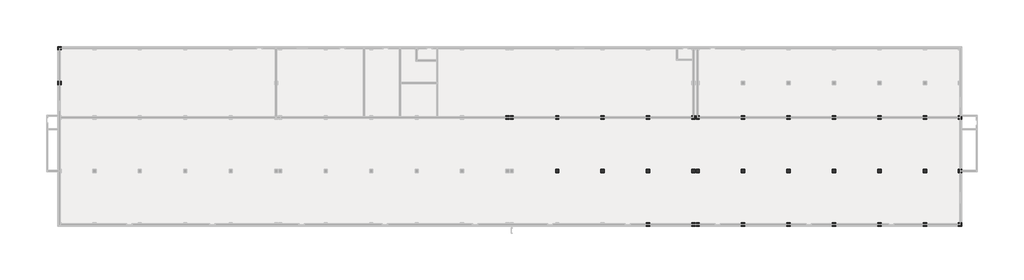
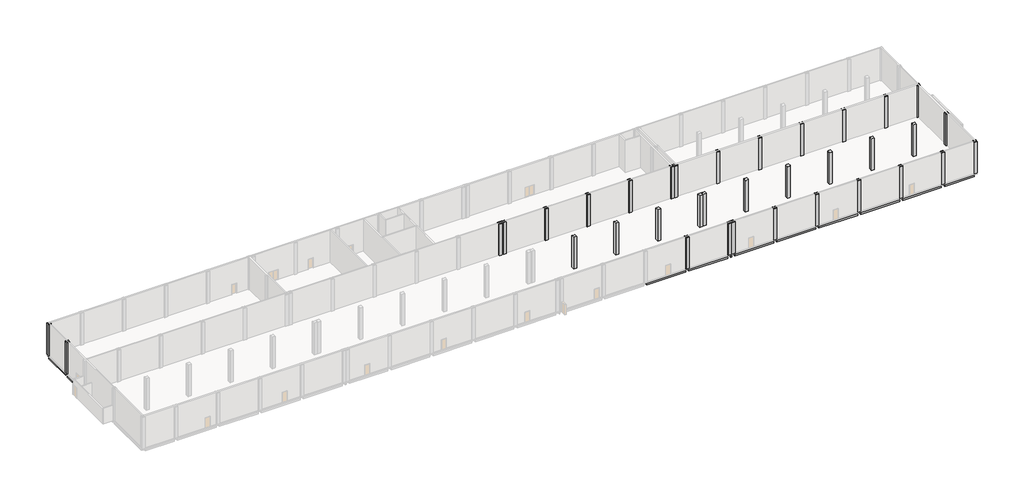
# One storey, part 3 of 4: 35 columns, 13 beams.
"""IFC4 building model written with IfcOpenShell, lengths in millimetres."""

from ifc_helpers import new_model, si_unit, frame, origin, place, context, project, spatial, polyline, outline, extrude, faceted_brep, element, save

model = new_model("IFC4")

# Units and contexts
model_context = context("Model", 3, world=origin())
ifc_project = project(units=[si_unit("LENGTHUNIT", "METRE", prefix="MILLI")], contexts=[model_context])

# Site, building, storey
site = spatial("IfcSite", under=ifc_project)
building = spatial("IfcBuilding", under=site)
storey = spatial("IfcBuildingStorey", under=building, Name="01_T.O.F", Elevation=299.9618634)

# Beams
placement = place(None, origin())
element("IfcBeam", 1, ObjectType="RC Beam_Rectangular : H_SB_AR_S16_TG_B400xH600", at=placement, inside=storey, context=model_context, shape_type="SweptSolid", body=[
    extrude(outline(polyline([(157955.0, -6300.4791411), (158305.0, -6300.4791411), (158305.0, -15350.4791411), (157955.0, -15350.4791411), (157955.0, -6300.4791411)])), frame((0.0, 0.0, -300.0381366), z_axis=(0.0, 0.0, 1.0), x_axis=(1.0, 0.0, 0.0)), (0.0, 0.0, 1.0), 450.0),
])
element("IfcBeam", 2, ObjectType="RC Beam_Rectangular : H_SB_AR_S16_TG_B400xH600", at=placement, inside=storey, context=model_context, shape_type="SweptSolid", body=[
    extrude(outline(polyline([(157955.0, -15950.4791411), (158305.0, -15950.4791411), (158305.0, -25000.4791411), (157955.0, -25000.4791411), (157955.0, -15950.4791411)])), frame((0.0, 0.0, -300.0381366), z_axis=(0.0, 0.0, 1.0), x_axis=(1.0, 0.0, 0.0)), (0.0, 0.0, 1.0), 450.0),
])
element("IfcBeam", 3, ObjectType="RC Beam_Rectangular : H_SB_AR_S16_TG_B400xH600", at=placement, inside=storey, context=model_context, shape_type="SweptSolid", body=[
    extrude(outline(polyline([(-4195.0, 549.5208589), (-4545.0, 549.5208589), (-4545.0, 6199.5208589), (-4195.0, 6199.5208589), (-4195.0, 549.5208589)])), frame((0.0, 0.0, -300.0381366), z_axis=(0.0, 0.0, 1.0), x_axis=(1.0, 0.0, 0.0)), (0.0, 0.0, 1.0), 450.0),
])
element("IfcBeam", 4, ObjectType="RC Beam_Rectangular : H_SB_AR_S16_TG_B400xH600", at=placement, inside=storey, context=model_context, shape_type="SweptSolid", body=[
    extrude(outline(polyline([(-4545.0, -50.4791411), (-4195.0, -50.4791411), (-4195.0, -5700.4791411), (-4545.0, -5700.4791411), (-4545.0, -50.4791411)])), frame((0.0, 0.0, -300.0381366), z_axis=(0.0, 0.0, 1.0), x_axis=(1.0, 0.0, 0.0)), (0.0, 0.0, 1.0), 450.0),
])
element("IfcBeam", 5, ObjectType="RC Beam_Rectangular : H_SB_AR_S16_TG_B400xH600", at=placement, inside=storey, context=model_context, shape_type="SweptSolid", body=[
    extrude(outline(polyline([(93930.0, -25475.4791411), (93930.0, -25125.4791411), (101530.0, -25125.4791411), (101530.0, -25475.4791411), (93930.0, -25475.4791411)])), frame((0.0, 0.0, -300.0381366), z_axis=(0.0, 0.0, 1.0), x_axis=(1.0, 0.0, 0.0)), (0.0, 0.0, 1.0), 450.0),
])
element("IfcBeam", 6, ObjectType="RC Beam_Rectangular : H_SB_AR_S16_TG_B400xH600", at=placement, inside=storey, context=model_context, shape_type="SweptSolid", body=[
    extrude(outline(polyline([(102130.0, -25475.4791411), (102130.0, -25125.4791411), (109730.0, -25125.4791411), (109730.0, -25475.4791411), (102130.0, -25475.4791411)])), frame((0.0, 0.0, -300.0381366), z_axis=(0.0, 0.0, 1.0), x_axis=(1.0, 0.0, 0.0)), (0.0, 0.0, 1.0), 450.0),
])
element("IfcBeam", 7, ObjectType="RC Beam_Rectangular : H_SB_AR_S16_TG_B400xH600", at=placement, inside=storey, context=model_context, shape_type="SweptSolid", body=[
    extrude(outline(polyline([(110330.0, -25475.4791411), (110330.0, -25125.4791411), (110480.0, -25125.4791411), (110480.0, -25475.4791411), (110330.0, -25475.4791411)])), frame((0.0, 0.0, -300.0381366), z_axis=(0.0, 0.0, 1.0), x_axis=(1.0, 0.0, 0.0)), (0.0, 0.0, 1.0), 450.0),
])
element("IfcBeam", 8, ObjectType="RC Beam_Rectangular : H_SB_AR_S16_TG_B400xH600", at=placement, inside=storey, context=model_context, shape_type="SweptSolid", body=[
    extrude(outline(polyline([(111080.0, -25475.4791411), (111080.0, -25125.4791411), (118680.0, -25125.4791411), (118680.0, -25475.4791411), (111080.0, -25475.4791411)])), frame((0.0, 0.0, -300.0381366), z_axis=(0.0, 0.0, 1.0), x_axis=(1.0, 0.0, 0.0)), (0.0, 0.0, 1.0), 450.0),
])
element("IfcBeam", 9, ObjectType="RC Beam_Rectangular : H_SB_AR_S16_TG_B400xH600", at=placement, inside=storey, context=model_context, shape_type="SweptSolid", body=[
    extrude(outline(polyline([(119280.0, -25475.4791411), (119280.0, -25125.4791411), (126880.0, -25125.4791411), (126880.0, -25475.4791411), (119280.0, -25475.4791411)])), frame((0.0, 0.0, -300.0381366), z_axis=(0.0, 0.0, 1.0), x_axis=(1.0, 0.0, 0.0)), (0.0, 0.0, 1.0), 450.0),
])
element("IfcBeam", 10, ObjectType="RC Beam_Rectangular : H_SB_AR_S16_TG_B400xH600", at=placement, inside=storey, context=model_context, shape_type="SweptSolid", body=[
    extrude(outline(polyline([(127480.0, -25475.4791411), (127480.0, -25125.4791411), (135080.0, -25125.4791411), (135080.0, -25475.4791411), (127480.0, -25475.4791411)])), frame((0.0, 0.0, -300.0381366), z_axis=(0.0, 0.0, 1.0), x_axis=(1.0, 0.0, 0.0)), (0.0, 0.0, 1.0), 450.0),
])
element("IfcBeam", 11, ObjectType="RC Beam_Rectangular : H_SB_AR_S16_TG_B400xH600", at=placement, inside=storey, context=model_context, shape_type="SweptSolid", body=[
    extrude(outline(polyline([(135680.0, -25475.4791411), (135680.0, -25125.4791411), (143280.0, -25125.4791411), (143280.0, -25475.4791411), (135680.0, -25475.4791411)])), frame((0.0, 0.0, -300.0381366), z_axis=(0.0, 0.0, 1.0), x_axis=(1.0, 0.0, 0.0)), (0.0, 0.0, 1.0), 450.0),
])
element("IfcBeam", 12, ObjectType="RC Beam_Rectangular : H_SB_AR_S16_TG_B400xH600", at=placement, inside=storey, context=model_context, shape_type="SweptSolid", body=[
    extrude(outline(polyline([(143880.0, -25475.4791411), (143880.0, -25125.4791411), (151480.0, -25125.4791411), (151480.0, -25475.4791411), (143880.0, -25475.4791411)])), frame((0.0, 0.0, -300.0381366), z_axis=(0.0, 0.0, 1.0), x_axis=(1.0, 0.0, 0.0)), (0.0, 0.0, 1.0), 450.0),
])
element("IfcBeam", 13, ObjectType="RC Beam_Rectangular : H_SB_AR_S16_TG_B400xH600", at=placement, inside=storey, context=model_context, shape_type="SweptSolid", body=[
    extrude(outline(polyline([(152080.0, -25475.4791411), (152080.0, -25125.4791411), (157830.0, -25125.4791411), (157830.0, -25475.4791411), (152080.0, -25475.4791411)])), frame((0.0, 0.0, -300.0381366), z_axis=(0.0, 0.0, 1.0), x_axis=(1.0, 0.0, 0.0)), (0.0, 0.0, 1.0), 450.0),
])

# Columns
element("IfcColumn", 14, ObjectType="RC_Column_Rectangular : H_SC_AR_S15_W600xL600", at=placement, inside=storey, context=model_context, shape_type="Brep", body=[
    faceted_brep([(-4070.0, 549.5208589, 299.9618634), (-4070.0, -50.4791411, 299.9618634), (-4670.0, -50.4791411, 299.9618634), (-4670.0, 549.5208589, 299.9618634), (-4070.0, 549.5208589, 6848.9618634), (-4070.0, 399.5208589, 6848.9618634), (-4070.0, 99.5208589, 6848.9618634), (-4070.0, -50.4791411, 6848.9618634), (-4220.0, -50.4791411, 6848.9618634), (-4520.0, -50.4791411, 6848.9618634), (-4670.0, -50.4791411, 6848.9618634), (-4670.0, 549.5208589, 6848.9618634), (-4520.0, 549.5208589, 6848.9618634), (-4220.0, 549.5208589, 6848.9618634)], [[[0, 1, 2, 3]], [[1, 0, 4, 5, 6, 7]], [[2, 1, 7, 8, 9, 10]], [[3, 2, 10, 11]], [[0, 3, 11, 12, 13, 4]], [[7, 6, 5, 4, 13, 12, 11, 10, 9, 8]]]),
])
element("IfcColumn", 15, ObjectType="RC_Column_Rectangular : H_SC_AR_S15_W600xL600", at=placement, inside=storey, context=model_context, shape_type="Brep", body=[
    faceted_brep([(-4070.0, 6799.5208589, 299.9618634), (-4070.0, 6199.5208589, 299.9618634), (-4670.0, 6199.5208589, 299.9618634), (-4670.0, 6799.5208589, 299.9618634), (-4070.0, 6799.5208589, 6848.9618634), (-4070.0, 6649.5208589, 6848.9618634), (-4070.0, 6349.5208589, 6848.9618634), (-4070.0, 6199.5208589, 6848.9618634), (-4220.0, 6199.5208589, 6848.9618634), (-4520.0, 6199.5208589, 6848.9618634), (-4670.0, 6199.5208589, 6848.9618634), (-4670.0, 6799.5208589, 6848.9618634)], [[[0, 1, 2, 3]], [[1, 0, 4, 5, 6, 7]], [[2, 1, 7, 8, 9, 10]], [[3, 2, 10, 11]], [[0, 3, 11, 4]], [[7, 6, 5, 4, 11, 10, 9, 8]]]),
])
element("IfcColumn", 16, ObjectType="RC_Column_Rectangular : H_SC_AR_S15_W600xL600", at=placement, inside=storey, context=model_context, shape_type="Brep", body=[
    faceted_brep([(76780.0, -5700.4791411, 299.9618634), (76780.0, -6300.4791411, 299.9618634), (76180.0, -6300.4791411, 299.9618634), (76180.0, -5700.4791411, 299.9618634), (76780.0, -5700.4791411, 6848.9618634), (76780.0, -5850.4791411, 6848.9618634), (76780.0, -6150.4791411, 6848.9618634), (76780.0, -6300.4791411, 6848.9618634), (76630.0, -6300.4791411, 6848.9618634), (76330.0, -6300.4791411, 6848.9618634), (76180.0, -6300.4791411, 6848.9618634), (76180.0, -6150.4791411, 6848.9618634), (76180.0, -5850.4791411, 6848.9618634), (76180.0, -5700.4791411, 6848.9618634), (76330.0, -5700.4791411, 6848.9618634), (76630.0, -5700.4791411, 6848.9618634)], [[[0, 1, 2, 3]], [[1, 0, 4, 5, 6, 7]], [[2, 1, 7, 8, 9, 10]], [[3, 2, 10, 11, 12, 13]], [[0, 3, 13, 14, 15, 4]], [[7, 6, 5, 4, 15, 14, 13, 12, 11, 10, 9, 8]]]),
])
element("IfcColumn", 17, ObjectType="RC_Column_Rectangular : H_SC_AR_S15_W600xL600", at=placement, inside=storey, context=model_context, shape_type="Brep", body=[
    faceted_brep([(77530.0, -5700.4791411, 299.9618634), (77530.0, -6300.4791411, 299.9618634), (76930.0, -6300.4791411, 299.9618634), (76930.0, -5700.4791411, 299.9618634), (77530.0, -5700.4791411, 6848.9618634), (77530.0, -5850.4791411, 6848.9618634), (77530.0, -6150.4791411, 6848.9618634), (77530.0, -6300.4791411, 6848.9618634), (77380.0, -6300.4791411, 6848.9618634), (77080.0, -6300.4791411, 6848.9618634), (76930.0, -6300.4791411, 6848.9618634), (76930.0, -6150.4791411, 6848.9618634), (76930.0, -5850.4791411, 6848.9618634), (76930.0, -5700.4791411, 6848.9618634), (77080.0, -5700.4791411, 6848.9618634), (77380.0, -5700.4791411, 6848.9618634)], [[[0, 1, 2, 3]], [[1, 0, 4, 5, 6, 7]], [[2, 1, 7, 8, 9, 10]], [[3, 2, 10, 11, 12, 13]], [[0, 3, 13, 14, 15, 4]], [[7, 6, 5, 4, 15, 14, 13, 12, 11, 10, 9, 8]]]),
])
element("IfcColumn", 18, ObjectType="RC_Column_Rectangular : H_SC_AR_S15_W600xL600", at=placement, inside=storey, context=model_context, shape_type="Brep", body=[
    faceted_brep([(85730.0, -5700.4791411, 299.9618634), (85730.0, -6300.4791411, 299.9618634), (85130.0, -6300.4791411, 299.9618634), (85130.0, -5700.4791411, 299.9618634), (85730.0, -5700.4791411, 6848.9618634), (85730.0, -5850.4791411, 6848.9618634), (85730.0, -6150.4791411, 6848.9618634), (85730.0, -6300.4791411, 6848.9618634), (85580.0, -6300.4791411, 6848.9618634), (85280.0, -6300.4791411, 6848.9618634), (85130.0, -6300.4791411, 6848.9618634), (85130.0, -6150.4791411, 6848.9618634), (85130.0, -5850.4791411, 6848.9618634), (85130.0, -5700.4791411, 6848.9618634), (85280.0, -5700.4791411, 6848.9618634), (85580.0, -5700.4791411, 6848.9618634)], [[[0, 1, 2, 3]], [[1, 0, 4, 5, 6, 7]], [[2, 1, 7, 8, 9, 10]], [[3, 2, 10, 11, 12, 13]], [[0, 3, 13, 14, 15, 4]], [[7, 6, 5, 4, 15, 14, 13, 12, 11, 10, 9, 8]]]),
])
element("IfcColumn", 19, ObjectType="RC_Column_Rectangular : H_SC_AR_S15_W600xL600", at=placement, inside=storey, context=model_context, shape_type="Brep", body=[
    faceted_brep([(93930.0, -5700.4791411, 299.9618634), (93930.0, -6300.4791411, 299.9618634), (93330.0, -6300.4791411, 299.9618634), (93330.0, -5700.4791411, 299.9618634), (93930.0, -5700.4791411, 6848.9618634), (93930.0, -5850.4791411, 6848.9618634), (93930.0, -6150.4791411, 6848.9618634), (93930.0, -6300.4791411, 6848.9618634), (93780.0, -6300.4791411, 6848.9618634), (93480.0, -6300.4791411, 6848.9618634), (93330.0, -6300.4791411, 6848.9618634), (93330.0, -6150.4791411, 6848.9618634), (93330.0, -5850.4791411, 6848.9618634), (93330.0, -5700.4791411, 6848.9618634), (93480.0, -5700.4791411, 6848.9618634), (93780.0, -5700.4791411, 6848.9618634)], [[[0, 1, 2, 3]], [[1, 0, 4, 5, 6, 7]], [[2, 1, 7, 8, 9, 10]], [[3, 2, 10, 11, 12, 13]], [[0, 3, 13, 14, 15, 4]], [[7, 6, 5, 4, 15, 14, 13, 12, 11, 10, 9, 8]]]),
])
element("IfcColumn", 20, ObjectType="RC_Column_Rectangular : H_SC_AR_S15_W600xL600", at=placement, inside=storey, context=model_context, shape_type="Brep", body=[
    faceted_brep([(102130.0, -5700.4791411, 299.9618634), (102130.0, -6300.4791411, 299.9618634), (101530.0, -6300.4791411, 299.9618634), (101530.0, -5700.4791411, 299.9618634), (102130.0, -5700.4791411, 6848.9618634), (102130.0, -5850.4791411, 6848.9618634), (102130.0, -6150.4791411, 6848.9618634), (102130.0, -6300.4791411, 6848.9618634), (101980.0, -6300.4791411, 6848.9618634), (101680.0, -6300.4791411, 6848.9618634), (101530.0, -6300.4791411, 6848.9618634), (101530.0, -6150.4791411, 6848.9618634), (101530.0, -5850.4791411, 6848.9618634), (101530.0, -5700.4791411, 6848.9618634), (101680.0, -5700.4791411, 6848.9618634), (101980.0, -5700.4791411, 6848.9618634)], [[[0, 1, 2, 3]], [[1, 0, 4, 5, 6, 7]], [[2, 1, 7, 8, 9, 10]], [[3, 2, 10, 11, 12, 13]], [[0, 3, 13, 14, 15, 4]], [[7, 6, 5, 4, 15, 14, 13, 12, 11, 10, 9, 8]]]),
])
element("IfcColumn", 21, ObjectType="RC_Column_Rectangular : H_SC_AR_S15_W600xL600", at=placement, inside=storey, context=model_context, shape_type="Brep", body=[
    faceted_brep([(110330.0, -5700.4791411, 299.9618634), (110330.0, -6300.4791411, 299.9618634), (109730.0, -6300.4791411, 299.9618634), (109730.0, -5700.4791411, 299.9618634), (110330.0, -5700.4791411, 6848.9618634), (110330.0, -5850.4791411, 6848.9618634), (110330.0, -6150.4791411, 6848.9618634), (110330.0, -6300.4791411, 6848.9618634), (110180.0, -6300.4791411, 6848.9618634), (109880.0, -6300.4791411, 6848.9618634), (109730.0, -6300.4791411, 6848.9618634), (109730.0, -6150.4791411, 6848.9618634), (109730.0, -5850.4791411, 6848.9618634), (109730.0, -5700.4791411, 6848.9618634), (109880.0, -5700.4791411, 6848.9618634), (110180.0, -5700.4791411, 6848.9618634)], [[[0, 1, 2, 3]], [[1, 0, 4, 5, 6, 7]], [[2, 1, 7, 8, 9, 10]], [[3, 2, 10, 11, 12, 13]], [[0, 3, 13, 14, 15, 4]], [[7, 6, 5, 4, 15, 14, 13, 12, 11, 10, 9, 8]]]),
])
element("IfcColumn", 22, ObjectType="RC_Column_Rectangular : H_SC_AR_S15_W600xL600", at=placement, inside=storey, context=model_context, shape_type="Brep", body=[
    faceted_brep([(111080.0, -5700.4791411, 299.9618634), (111080.0, -6300.4791411, 299.9618634), (110480.0, -6300.4791411, 299.9618634), (110480.0, -5700.4791411, 299.9618634), (111080.0, -5700.4791411, 6848.9618634), (111080.0, -5850.4791411, 6848.9618634), (111080.0, -6150.4791411, 6848.9618634), (111080.0, -6300.4791411, 6848.9618634), (110930.0, -6300.4791411, 6848.9618634), (110630.0, -6300.4791411, 6848.9618634), (110480.0, -6300.4791411, 6848.9618634), (110480.0, -6150.4791411, 6848.9618634), (110480.0, -5850.4791411, 6848.9618634), (110480.0, -5700.4791411, 6848.9618634), (110630.0, -5700.4791411, 6848.9618634), (110930.0, -5700.4791411, 6848.9618634)], [[[0, 1, 2, 3]], [[1, 0, 4, 5, 6, 7]], [[2, 1, 7, 8, 9, 10]], [[3, 2, 10, 11, 12, 13]], [[0, 3, 13, 14, 15, 4]], [[7, 6, 5, 4, 15, 14, 13, 12, 11, 10, 9, 8]]]),
])
element("IfcColumn", 23, ObjectType="RC_Column_Rectangular : H_SC_AR_S15_W600xL600", at=placement, inside=storey, context=model_context, shape_type="Brep", body=[
    faceted_brep([(119280.0, -5700.4791411, 299.9618634), (119280.0, -6300.4791411, 299.9618634), (118680.0, -6300.4791411, 299.9618634), (118680.0, -5700.4791411, 299.9618634), (119280.0, -5700.4791411, 6848.9618634), (119280.0, -5850.4791411, 6848.9618634), (119280.0, -6150.4791411, 6848.9618634), (119280.0, -6300.4791411, 6848.9618634), (119130.0, -6300.4791411, 6848.9618634), (118830.0, -6300.4791411, 6848.9618634), (118680.0, -6300.4791411, 6848.9618634), (118680.0, -6150.4791411, 6848.9618634), (118680.0, -5850.4791411, 6848.9618634), (118680.0, -5700.4791411, 6848.9618634), (118830.0, -5700.4791411, 6848.9618634), (119130.0, -5700.4791411, 6848.9618634)], [[[0, 1, 2, 3]], [[1, 0, 4, 5, 6, 7]], [[2, 1, 7, 8, 9, 10]], [[3, 2, 10, 11, 12, 13]], [[0, 3, 13, 14, 15, 4]], [[7, 6, 5, 4, 15, 14, 13, 12, 11, 10, 9, 8]]]),
])
element("IfcColumn", 24, ObjectType="RC_Column_Rectangular : H_SC_AR_S15_W600xL600", at=placement, inside=storey, context=model_context, shape_type="Brep", body=[
    faceted_brep([(127480.0, -5700.4791411, 299.9618634), (127480.0, -6300.4791411, 299.9618634), (126880.0, -6300.4791411, 299.9618634), (126880.0, -5700.4791411, 299.9618634), (127480.0, -5700.4791411, 6848.9618634), (127480.0, -5850.4791411, 6848.9618634), (127480.0, -6150.4791411, 6848.9618634), (127480.0, -6300.4791411, 6848.9618634), (127330.0, -6300.4791411, 6848.9618634), (127030.0, -6300.4791411, 6848.9618634), (126880.0, -6300.4791411, 6848.9618634), (126880.0, -6150.4791411, 6848.9618634), (126880.0, -5850.4791411, 6848.9618634), (126880.0, -5700.4791411, 6848.9618634), (127030.0, -5700.4791411, 6848.9618634), (127330.0, -5700.4791411, 6848.9618634)], [[[0, 1, 2, 3]], [[1, 0, 4, 5, 6, 7]], [[2, 1, 7, 8, 9, 10]], [[3, 2, 10, 11, 12, 13]], [[0, 3, 13, 14, 15, 4]], [[7, 6, 5, 4, 15, 14, 13, 12, 11, 10, 9, 8]]]),
])
element("IfcColumn", 25, ObjectType="RC_Column_Rectangular : H_SC_AR_S15_W600xL600", at=placement, inside=storey, context=model_context, shape_type="Brep", body=[
    faceted_brep([(135680.0, -5700.4791411, 299.9618634), (135680.0, -6300.4791411, 299.9618634), (135080.0, -6300.4791411, 299.9618634), (135080.0, -5700.4791411, 299.9618634), (135680.0, -5700.4791411, 6848.9618634), (135680.0, -5850.4791411, 6848.9618634), (135680.0, -6150.4791411, 6848.9618634), (135680.0, -6300.4791411, 6848.9618634), (135530.0, -6300.4791411, 6848.9618634), (135230.0, -6300.4791411, 6848.9618634), (135080.0, -6300.4791411, 6848.9618634), (135080.0, -6150.4791411, 6848.9618634), (135080.0, -5850.4791411, 6848.9618634), (135080.0, -5700.4791411, 6848.9618634), (135230.0, -5700.4791411, 6848.9618634), (135530.0, -5700.4791411, 6848.9618634)], [[[0, 1, 2, 3]], [[1, 0, 4, 5, 6, 7]], [[2, 1, 7, 8, 9, 10]], [[3, 2, 10, 11, 12, 13]], [[0, 3, 13, 14, 15, 4]], [[7, 6, 5, 4, 15, 14, 13, 12, 11, 10, 9, 8]]]),
])
element("IfcColumn", 26, ObjectType="RC_Column_Rectangular : H_SC_AR_S15_W600xL600", at=placement, inside=storey, context=model_context, shape_type="Brep", body=[
    faceted_brep([(143880.0, -5700.4791411, 299.9618634), (143880.0, -6300.4791411, 299.9618634), (143280.0, -6300.4791411, 299.9618634), (143280.0, -5700.4791411, 299.9618634), (143880.0, -5700.4791411, 6848.9618634), (143880.0, -5850.4791411, 6848.9618634), (143880.0, -6150.4791411, 6848.9618634), (143880.0, -6300.4791411, 6848.9618634), (143730.0, -6300.4791411, 6848.9618634), (143430.0, -6300.4791411, 6848.9618634), (143280.0, -6300.4791411, 6848.9618634), (143280.0, -6150.4791411, 6848.9618634), (143280.0, -5850.4791411, 6848.9618634), (143280.0, -5700.4791411, 6848.9618634), (143430.0, -5700.4791411, 6848.9618634), (143730.0, -5700.4791411, 6848.9618634)], [[[0, 1, 2, 3]], [[1, 0, 4, 5, 6, 7]], [[2, 1, 7, 8, 9, 10]], [[3, 2, 10, 11, 12, 13]], [[0, 3, 13, 14, 15, 4]], [[7, 6, 5, 4, 15, 14, 13, 12, 11, 10, 9, 8]]]),
])
element("IfcColumn", 27, ObjectType="RC_Column_Rectangular : H_SC_AR_S15_W600xL600", at=placement, inside=storey, context=model_context, shape_type="Brep", body=[
    faceted_brep([(152080.0, -5700.4791411, 299.9618634), (152080.0, -6300.4791411, 299.9618634), (151480.0, -6300.4791411, 299.9618634), (151480.0, -5700.4791411, 299.9618634), (152080.0, -5700.4791411, 6848.9618634), (152080.0, -5850.4791411, 6848.9618634), (152080.0, -6150.4791411, 6848.9618634), (152080.0, -6300.4791411, 6848.9618634), (151930.0, -6300.4791411, 6848.9618634), (151630.0, -6300.4791411, 6848.9618634), (151480.0, -6300.4791411, 6848.9618634), (151480.0, -6150.4791411, 6848.9618634), (151480.0, -5850.4791411, 6848.9618634), (151480.0, -5700.4791411, 6848.9618634), (151630.0, -5700.4791411, 6848.9618634), (151930.0, -5700.4791411, 6848.9618634)], [[[0, 1, 2, 3]], [[1, 0, 4, 5, 6, 7]], [[2, 1, 7, 8, 9, 10]], [[3, 2, 10, 11, 12, 13]], [[0, 3, 13, 14, 15, 4]], [[7, 6, 5, 4, 15, 14, 13, 12, 11, 10, 9, 8]]]),
])
element("IfcColumn", 28, ObjectType="RC_Column_Rectangular : H_SC_AR_S15_W600xL600", at=placement, inside=storey, context=model_context, shape_type="Brep", body=[
    faceted_brep([(158430.0, -5700.4791411, 299.9618634), (158430.0, -6300.4791411, 299.9618634), (157830.0, -6300.4791411, 299.9618634), (157830.0, -5700.4791411, 299.9618634), (158430.0, -5700.4791411, 6848.9618634), (158430.0, -6300.4791411, 6848.9618634), (158280.0, -6300.4791411, 6848.9618634), (157980.0, -6300.4791411, 6848.9618634), (157830.0, -6300.4791411, 6848.9618634), (157830.0, -6150.4791411, 6848.9618634), (157830.0, -5850.4791411, 6848.9618634), (157830.0, -5700.4791411, 6848.9618634), (157980.0, -5700.4791411, 6848.9618634), (158280.0, -5700.4791411, 6848.9618634)], [[[0, 1, 2, 3]], [[1, 0, 4, 5]], [[2, 1, 5, 6, 7, 8]], [[3, 2, 8, 9, 10, 11]], [[0, 3, 11, 12, 13, 4]], [[5, 4, 13, 12, 11, 10, 9, 8, 7, 6]]]),
])
element("IfcColumn", 29, ObjectType="RC_Column_Rectangular : H_SC_AR_S15_W600xL600", at=placement, inside=storey, context=model_context, shape_type="Brep", body=[
    faceted_brep([(85730.0, -15350.4791411, 299.9618634), (85730.0, -15950.4791411, 299.9618634), (85130.0, -15950.4791411, 299.9618634), (85130.0, -15350.4791411, 299.9618634), (85730.0, -15350.4791411, 6848.9618634), (85730.0, -15500.4791411, 6848.9618634), (85730.0, -15800.4791411, 6848.9618634), (85730.0, -15950.4791411, 6848.9618634), (85580.0, -15950.4791411, 6848.9618634), (85280.0, -15950.4791411, 6848.9618634), (85130.0, -15950.4791411, 6848.9618634), (85130.0, -15800.4791411, 6848.9618634), (85130.0, -15500.4791411, 6848.9618634), (85130.0, -15350.4791411, 6848.9618634), (85280.0, -15350.4791411, 6848.9618634), (85580.0, -15350.4791411, 6848.9618634)], [[[0, 1, 2, 3]], [[1, 0, 4, 5, 6, 7]], [[2, 1, 7, 8, 9, 10]], [[3, 2, 10, 11, 12, 13]], [[0, 3, 13, 14, 15, 4]], [[7, 6, 5, 4, 15, 14, 13, 12, 11, 10, 9, 8]]]),
])
element("IfcColumn", 30, ObjectType="RC_Column_Rectangular : H_SC_AR_S15_W600xL600", at=placement, inside=storey, context=model_context, shape_type="Brep", body=[
    faceted_brep([(93930.0, -15350.4791411, 299.9618634), (93930.0, -15950.4791411, 299.9618634), (93330.0, -15950.4791411, 299.9618634), (93330.0, -15350.4791411, 299.9618634), (93930.0, -15350.4791411, 6848.9618634), (93930.0, -15500.4791411, 6848.9618634), (93930.0, -15800.4791411, 6848.9618634), (93930.0, -15950.4791411, 6848.9618634), (93780.0, -15950.4791411, 6848.9618634), (93480.0, -15950.4791411, 6848.9618634), (93330.0, -15950.4791411, 6848.9618634), (93330.0, -15800.4791411, 6848.9618634), (93330.0, -15500.4791411, 6848.9618634), (93330.0, -15350.4791411, 6848.9618634), (93480.0, -15350.4791411, 6848.9618634), (93780.0, -15350.4791411, 6848.9618634)], [[[0, 1, 2, 3]], [[1, 0, 4, 5, 6, 7]], [[2, 1, 7, 8, 9, 10]], [[3, 2, 10, 11, 12, 13]], [[0, 3, 13, 14, 15, 4]], [[7, 6, 5, 4, 15, 14, 13, 12, 11, 10, 9, 8]]]),
])
element("IfcColumn", 31, ObjectType="RC_Column_Rectangular : H_SC_AR_S15_W600xL600", at=placement, inside=storey, context=model_context, shape_type="Brep", body=[
    faceted_brep([(102130.0, -15350.4791411, 299.9618634), (102130.0, -15950.4791411, 299.9618634), (101530.0, -15950.4791411, 299.9618634), (101530.0, -15350.4791411, 299.9618634), (102130.0, -15350.4791411, 6848.9618634), (102130.0, -15500.4791411, 6848.9618634), (102130.0, -15800.4791411, 6848.9618634), (102130.0, -15950.4791411, 6848.9618634), (101980.0, -15950.4791411, 6848.9618634), (101680.0, -15950.4791411, 6848.9618634), (101530.0, -15950.4791411, 6848.9618634), (101530.0, -15800.4791411, 6848.9618634), (101530.0, -15500.4791411, 6848.9618634), (101530.0, -15350.4791411, 6848.9618634), (101680.0, -15350.4791411, 6848.9618634), (101980.0, -15350.4791411, 6848.9618634)], [[[0, 1, 2, 3]], [[1, 0, 4, 5, 6, 7]], [[2, 1, 7, 8, 9, 10]], [[3, 2, 10, 11, 12, 13]], [[0, 3, 13, 14, 15, 4]], [[7, 6, 5, 4, 15, 14, 13, 12, 11, 10, 9, 8]]]),
])
element("IfcColumn", 32, ObjectType="RC_Column_Rectangular : H_SC_AR_S15_W600xL600", at=placement, inside=storey, context=model_context, shape_type="Brep", body=[
    faceted_brep([(110330.0, -15350.4791411, 299.9618634), (110330.0, -15950.4791411, 299.9618634), (109730.0, -15950.4791411, 299.9618634), (109730.0, -15350.4791411, 299.9618634), (110330.0, -15350.4791411, 6848.9618634), (110330.0, -15500.4791411, 6848.9618634), (110330.0, -15800.4791411, 6848.9618634), (110330.0, -15950.4791411, 6848.9618634), (110180.0, -15950.4791411, 6848.9618634), (109880.0, -15950.4791411, 6848.9618634), (109730.0, -15950.4791411, 6848.9618634), (109730.0, -15800.4791411, 6848.9618634), (109730.0, -15500.4791411, 6848.9618634), (109730.0, -15350.4791411, 6848.9618634), (109880.0, -15350.4791411, 6848.9618634), (110180.0, -15350.4791411, 6848.9618634)], [[[0, 1, 2, 3]], [[1, 0, 4, 5, 6, 7]], [[2, 1, 7, 8, 9, 10]], [[3, 2, 10, 11, 12, 13]], [[0, 3, 13, 14, 15, 4]], [[7, 6, 5, 4, 15, 14, 13, 12, 11, 10, 9, 8]]]),
])
element("IfcColumn", 33, ObjectType="RC_Column_Rectangular : H_SC_AR_S15_W600xL600", at=placement, inside=storey, context=model_context, shape_type="Brep", body=[
    faceted_brep([(111080.0, -15350.4791411, 299.9618634), (111080.0, -15950.4791411, 299.9618634), (110480.0, -15950.4791411, 299.9618634), (110480.0, -15350.4791411, 299.9618634), (111080.0, -15350.4791411, 6848.9618634), (111080.0, -15500.4791411, 6848.9618634), (111080.0, -15800.4791411, 6848.9618634), (111080.0, -15950.4791411, 6848.9618634), (110930.0, -15950.4791411, 6848.9618634), (110630.0, -15950.4791411, 6848.9618634), (110480.0, -15950.4791411, 6848.9618634), (110480.0, -15800.4791411, 6848.9618634), (110480.0, -15500.4791411, 6848.9618634), (110480.0, -15350.4791411, 6848.9618634), (110630.0, -15350.4791411, 6848.9618634), (110930.0, -15350.4791411, 6848.9618634)], [[[0, 1, 2, 3]], [[1, 0, 4, 5, 6, 7]], [[2, 1, 7, 8, 9, 10]], [[3, 2, 10, 11, 12, 13]], [[0, 3, 13, 14, 15, 4]], [[7, 6, 5, 4, 15, 14, 13, 12, 11, 10, 9, 8]]]),
])
element("IfcColumn", 34, ObjectType="RC_Column_Rectangular : H_SC_AR_S15_W600xL600", at=placement, inside=storey, context=model_context, shape_type="Brep", body=[
    faceted_brep([(119280.0, -15350.4791411, 299.9618634), (119280.0, -15950.4791411, 299.9618634), (118680.0, -15950.4791411, 299.9618634), (118680.0, -15350.4791411, 299.9618634), (119280.0, -15350.4791411, 6848.9618634), (119280.0, -15500.4791411, 6848.9618634), (119280.0, -15800.4791411, 6848.9618634), (119280.0, -15950.4791411, 6848.9618634), (119130.0, -15950.4791411, 6848.9618634), (118830.0, -15950.4791411, 6848.9618634), (118680.0, -15950.4791411, 6848.9618634), (118680.0, -15800.4791411, 6848.9618634), (118680.0, -15500.4791411, 6848.9618634), (118680.0, -15350.4791411, 6848.9618634), (118830.0, -15350.4791411, 6848.9618634), (119130.0, -15350.4791411, 6848.9618634)], [[[0, 1, 2, 3]], [[1, 0, 4, 5, 6, 7]], [[2, 1, 7, 8, 9, 10]], [[3, 2, 10, 11, 12, 13]], [[0, 3, 13, 14, 15, 4]], [[7, 6, 5, 4, 15, 14, 13, 12, 11, 10, 9, 8]]]),
])
element("IfcColumn", 35, ObjectType="RC_Column_Rectangular : H_SC_AR_S15_W600xL600", at=placement, inside=storey, context=model_context, shape_type="Brep", body=[
    faceted_brep([(127480.0, -15350.4791411, 299.9618634), (127480.0, -15950.4791411, 299.9618634), (126880.0, -15950.4791411, 299.9618634), (126880.0, -15350.4791411, 299.9618634), (127480.0, -15350.4791411, 6848.9618634), (127480.0, -15500.4791411, 6848.9618634), (127480.0, -15800.4791411, 6848.9618634), (127480.0, -15950.4791411, 6848.9618634), (127330.0, -15950.4791411, 6848.9618634), (127030.0, -15950.4791411, 6848.9618634), (126880.0, -15950.4791411, 6848.9618634), (126880.0, -15800.4791411, 6848.9618634), (126880.0, -15500.4791411, 6848.9618634), (126880.0, -15350.4791411, 6848.9618634), (127030.0, -15350.4791411, 6848.9618634), (127330.0, -15350.4791411, 6848.9618634)], [[[0, 1, 2, 3]], [[1, 0, 4, 5, 6, 7]], [[2, 1, 7, 8, 9, 10]], [[3, 2, 10, 11, 12, 13]], [[0, 3, 13, 14, 15, 4]], [[7, 6, 5, 4, 15, 14, 13, 12, 11, 10, 9, 8]]]),
])
element("IfcColumn", 36, ObjectType="RC_Column_Rectangular : H_SC_AR_S15_W600xL600", at=placement, inside=storey, context=model_context, shape_type="Brep", body=[
    faceted_brep([(135680.0, -15350.4791411, 299.9618634), (135680.0, -15950.4791411, 299.9618634), (135080.0, -15950.4791411, 299.9618634), (135080.0, -15350.4791411, 299.9618634), (135680.0, -15350.4791411, 6848.9618634), (135680.0, -15500.4791411, 6848.9618634), (135680.0, -15800.4791411, 6848.9618634), (135680.0, -15950.4791411, 6848.9618634), (135530.0, -15950.4791411, 6848.9618634), (135230.0, -15950.4791411, 6848.9618634), (135080.0, -15950.4791411, 6848.9618634), (135080.0, -15800.4791411, 6848.9618634), (135080.0, -15500.4791411, 6848.9618634), (135080.0, -15350.4791411, 6848.9618634), (135230.0, -15350.4791411, 6848.9618634), (135530.0, -15350.4791411, 6848.9618634)], [[[0, 1, 2, 3]], [[1, 0, 4, 5, 6, 7]], [[2, 1, 7, 8, 9, 10]], [[3, 2, 10, 11, 12, 13]], [[0, 3, 13, 14, 15, 4]], [[7, 6, 5, 4, 15, 14, 13, 12, 11, 10, 9, 8]]]),
])
element("IfcColumn", 37, ObjectType="RC_Column_Rectangular : H_SC_AR_S15_W600xL600", at=placement, inside=storey, context=model_context, shape_type="Brep", body=[
    faceted_brep([(143880.0, -15350.4791411, 299.9618634), (143880.0, -15950.4791411, 299.9618634), (143280.0, -15950.4791411, 299.9618634), (143280.0, -15350.4791411, 299.9618634), (143880.0, -15350.4791411, 6848.9618634), (143880.0, -15500.4791411, 6848.9618634), (143880.0, -15800.4791411, 6848.9618634), (143880.0, -15950.4791411, 6848.9618634), (143730.0, -15950.4791411, 6848.9618634), (143430.0, -15950.4791411, 6848.9618634), (143280.0, -15950.4791411, 6848.9618634), (143280.0, -15800.4791411, 6848.9618634), (143280.0, -15500.4791411, 6848.9618634), (143280.0, -15350.4791411, 6848.9618634), (143430.0, -15350.4791411, 6848.9618634), (143730.0, -15350.4791411, 6848.9618634)], [[[0, 1, 2, 3]], [[1, 0, 4, 5, 6, 7]], [[2, 1, 7, 8, 9, 10]], [[3, 2, 10, 11, 12, 13]], [[0, 3, 13, 14, 15, 4]], [[7, 6, 5, 4, 15, 14, 13, 12, 11, 10, 9, 8]]]),
])
element("IfcColumn", 38, ObjectType="RC_Column_Rectangular : H_SC_AR_S15_W600xL600", at=placement, inside=storey, context=model_context, shape_type="Brep", body=[
    faceted_brep([(152080.0, -15350.4791411, 299.9618634), (152080.0, -15950.4791411, 299.9618634), (151480.0, -15950.4791411, 299.9618634), (151480.0, -15350.4791411, 299.9618634), (152080.0, -15350.4791411, 6848.9618634), (152080.0, -15500.4791411, 6848.9618634), (152080.0, -15800.4791411, 6848.9618634), (152080.0, -15950.4791411, 6848.9618634), (151930.0, -15950.4791411, 6848.9618634), (151630.0, -15950.4791411, 6848.9618634), (151480.0, -15950.4791411, 6848.9618634), (151480.0, -15800.4791411, 6848.9618634), (151480.0, -15500.4791411, 6848.9618634), (151480.0, -15350.4791411, 6848.9618634), (151630.0, -15350.4791411, 6848.9618634), (151930.0, -15350.4791411, 6848.9618634)], [[[0, 1, 2, 3]], [[1, 0, 4, 5, 6, 7]], [[2, 1, 7, 8, 9, 10]], [[3, 2, 10, 11, 12, 13]], [[0, 3, 13, 14, 15, 4]], [[7, 6, 5, 4, 15, 14, 13, 12, 11, 10, 9, 8]]]),
])
element("IfcColumn", 39, ObjectType="RC_Column_Rectangular : H_SC_AR_S15_W600xL600", at=placement, inside=storey, context=model_context, shape_type="Brep", body=[
    faceted_brep([(158430.0, -15350.4791411, 299.9618634), (158430.0, -15950.4791411, 299.9618634), (157830.0, -15950.4791411, 299.9618634), (157830.0, -15350.4791411, 299.9618634), (158430.0, -15350.4791411, 6848.9618634), (158430.0, -15950.4791411, 6848.9618634), (158280.0, -15950.4791411, 6848.9618634), (157980.0, -15950.4791411, 6848.9618634), (157830.0, -15950.4791411, 6848.9618634), (157830.0, -15800.4791411, 6848.9618634), (157830.0, -15500.4791411, 6848.9618634), (157830.0, -15350.4791411, 6848.9618634), (157980.0, -15350.4791411, 6848.9618634), (158280.0, -15350.4791411, 6848.9618634)], [[[0, 1, 2, 3]], [[1, 0, 4, 5]], [[2, 1, 5, 6, 7, 8]], [[3, 2, 8, 9, 10, 11]], [[0, 3, 11, 12, 13, 4]], [[5, 4, 13, 12, 11, 10, 9, 8, 7, 6]]]),
])
element("IfcColumn", 40, ObjectType="RC_Column_Rectangular : H_SC_AR_S15_W600xL600", at=placement, inside=storey, context=model_context, shape_type="Brep", body=[
    faceted_brep([(102130.0, -25000.4791411, 299.9618634), (102130.0, -25600.4791411, 299.9618634), (101530.0, -25600.4791411, 299.9618634), (101530.0, -25000.4791411, 299.9618634), (102130.0, -25000.4791411, 6848.9618634), (102130.0, -25150.4791411, 6848.9618634), (102130.0, -25450.4791411, 6848.9618634), (102130.0, -25600.4791411, 6848.9618634), (101530.0, -25600.4791411, 6848.9618634), (101530.0, -25450.4791411, 6848.9618634), (101530.0, -25150.4791411, 6848.9618634), (101530.0, -25000.4791411, 6848.9618634), (101680.0, -25000.4791411, 6848.9618634), (101980.0, -25000.4791411, 6848.9618634)], [[[0, 1, 2, 3]], [[1, 0, 4, 5, 6, 7]], [[2, 1, 7, 8]], [[3, 2, 8, 9, 10, 11]], [[0, 3, 11, 12, 13, 4]], [[7, 6, 5, 4, 13, 12, 11, 10, 9, 8]]]),
])
element("IfcColumn", 41, ObjectType="RC_Column_Rectangular : H_SC_AR_S15_W600xL600", at=placement, inside=storey, context=model_context, shape_type="Brep", body=[
    faceted_brep([(110330.0, -25000.4791411, 299.9618634), (110330.0, -25600.4791411, 299.9618634), (109730.0, -25600.4791411, 299.9618634), (109730.0, -25000.4791411, 299.9618634), (110330.0, -25000.4791411, 6848.9618634), (110330.0, -25150.4791411, 6848.9618634), (110330.0, -25450.4791411, 6848.9618634), (110330.0, -25600.4791411, 6848.9618634), (109730.0, -25600.4791411, 6848.9618634), (109730.0, -25450.4791411, 6848.9618634), (109730.0, -25150.4791411, 6848.9618634), (109730.0, -25000.4791411, 6848.9618634), (109880.0, -25000.4791411, 6848.9618634), (110180.0, -25000.4791411, 6848.9618634)], [[[0, 1, 2, 3]], [[1, 0, 4, 5, 6, 7]], [[2, 1, 7, 8]], [[3, 2, 8, 9, 10, 11]], [[0, 3, 11, 12, 13, 4]], [[7, 6, 5, 4, 13, 12, 11, 10, 9, 8]]]),
])
element("IfcColumn", 42, ObjectType="RC_Column_Rectangular : H_SC_AR_S15_W600xL600", at=placement, inside=storey, context=model_context, shape_type="Brep", body=[
    faceted_brep([(111080.0, -25000.4791411, 299.9618634), (111080.0, -25600.4791411, 299.9618634), (110480.0, -25600.4791411, 299.9618634), (110480.0, -25000.4791411, 299.9618634), (111080.0, -25000.4791411, 6848.9618634), (111080.0, -25150.4791411, 6848.9618634), (111080.0, -25450.4791411, 6848.9618634), (111080.0, -25600.4791411, 6848.9618634), (110480.0, -25600.4791411, 6848.9618634), (110480.0, -25450.4791411, 6848.9618634), (110480.0, -25150.4791411, 6848.9618634), (110480.0, -25000.4791411, 6848.9618634), (110630.0, -25000.4791411, 6848.9618634), (110930.0, -25000.4791411, 6848.9618634)], [[[0, 1, 2, 3]], [[1, 0, 4, 5, 6, 7]], [[2, 1, 7, 8]], [[3, 2, 8, 9, 10, 11]], [[0, 3, 11, 12, 13, 4]], [[7, 6, 5, 4, 13, 12, 11, 10, 9, 8]]]),
])
element("IfcColumn", 43, ObjectType="RC_Column_Rectangular : H_SC_AR_S15_W600xL600", at=placement, inside=storey, context=model_context, shape_type="Brep", body=[
    faceted_brep([(119280.0, -25000.4791411, 299.9618634), (119280.0, -25600.4791411, 299.9618634), (118680.0, -25600.4791411, 299.9618634), (118680.0, -25000.4791411, 299.9618634), (119280.0, -25000.4791411, 6848.9618634), (119280.0, -25150.4791411, 6848.9618634), (119280.0, -25450.4791411, 6848.9618634), (119280.0, -25600.4791411, 6848.9618634), (118680.0, -25600.4791411, 6848.9618634), (118680.0, -25450.4791411, 6848.9618634), (118680.0, -25150.4791411, 6848.9618634), (118680.0, -25000.4791411, 6848.9618634), (118830.0, -25000.4791411, 6848.9618634), (119130.0, -25000.4791411, 6848.9618634)], [[[0, 1, 2, 3]], [[1, 0, 4, 5, 6, 7]], [[2, 1, 7, 8]], [[3, 2, 8, 9, 10, 11]], [[0, 3, 11, 12, 13, 4]], [[7, 6, 5, 4, 13, 12, 11, 10, 9, 8]]]),
])
element("IfcColumn", 44, ObjectType="RC_Column_Rectangular : H_SC_AR_S15_W600xL600", at=placement, inside=storey, context=model_context, shape_type="Brep", body=[
    faceted_brep([(127480.0, -25000.4791411, 299.9618634), (127480.0, -25600.4791411, 299.9618634), (126880.0, -25600.4791411, 299.9618634), (126880.0, -25000.4791411, 299.9618634), (127480.0, -25000.4791411, 6848.9618634), (127480.0, -25150.4791411, 6848.9618634), (127480.0, -25450.4791411, 6848.9618634), (127480.0, -25600.4791411, 6848.9618634), (126880.0, -25600.4791411, 6848.9618634), (126880.0, -25450.4791411, 6848.9618634), (126880.0, -25150.4791411, 6848.9618634), (126880.0, -25000.4791411, 6848.9618634), (127030.0, -25000.4791411, 6848.9618634), (127330.0, -25000.4791411, 6848.9618634)], [[[0, 1, 2, 3]], [[1, 0, 4, 5, 6, 7]], [[2, 1, 7, 8]], [[3, 2, 8, 9, 10, 11]], [[0, 3, 11, 12, 13, 4]], [[7, 6, 5, 4, 13, 12, 11, 10, 9, 8]]]),
])
element("IfcColumn", 45, ObjectType="RC_Column_Rectangular : H_SC_AR_S15_W600xL600", at=placement, inside=storey, context=model_context, shape_type="Brep", body=[
    faceted_brep([(135680.0, -25000.4791411, 299.9618634), (135680.0, -25600.4791411, 299.9618634), (135080.0, -25600.4791411, 299.9618634), (135080.0, -25000.4791411, 299.9618634), (135680.0, -25000.4791411, 6848.9618634), (135680.0, -25150.4791411, 6848.9618634), (135680.0, -25450.4791411, 6848.9618634), (135680.0, -25600.4791411, 6848.9618634), (135080.0, -25600.4791411, 6848.9618634), (135080.0, -25450.4791411, 6848.9618634), (135080.0, -25150.4791411, 6848.9618634), (135080.0, -25000.4791411, 6848.9618634), (135230.0, -25000.4791411, 6848.9618634), (135530.0, -25000.4791411, 6848.9618634)], [[[0, 1, 2, 3]], [[1, 0, 4, 5, 6, 7]], [[2, 1, 7, 8]], [[3, 2, 8, 9, 10, 11]], [[0, 3, 11, 12, 13, 4]], [[7, 6, 5, 4, 13, 12, 11, 10, 9, 8]]]),
])
element("IfcColumn", 46, ObjectType="RC_Column_Rectangular : H_SC_AR_S15_W600xL600", at=placement, inside=storey, context=model_context, shape_type="Brep", body=[
    faceted_brep([(143880.0, -25000.4791411, 299.9618634), (143880.0, -25600.4791411, 299.9618634), (143280.0, -25600.4791411, 299.9618634), (143280.0, -25000.4791411, 299.9618634), (143880.0, -25000.4791411, 6848.9618634), (143880.0, -25150.4791411, 6848.9618634), (143880.0, -25450.4791411, 6848.9618634), (143880.0, -25600.4791411, 6848.9618634), (143280.0, -25600.4791411, 6848.9618634), (143280.0, -25450.4791411, 6848.9618634), (143280.0, -25150.4791411, 6848.9618634), (143280.0, -25000.4791411, 6848.9618634), (143430.0, -25000.4791411, 6848.9618634), (143730.0, -25000.4791411, 6848.9618634)], [[[0, 1, 2, 3]], [[1, 0, 4, 5, 6, 7]], [[2, 1, 7, 8]], [[3, 2, 8, 9, 10, 11]], [[0, 3, 11, 12, 13, 4]], [[7, 6, 5, 4, 13, 12, 11, 10, 9, 8]]]),
])
element("IfcColumn", 47, ObjectType="RC_Column_Rectangular : H_SC_AR_S15_W600xL600", at=placement, inside=storey, context=model_context, shape_type="Brep", body=[
    faceted_brep([(152080.0, -25000.4791411, 299.9618634), (152080.0, -25600.4791411, 299.9618634), (151480.0, -25600.4791411, 299.9618634), (151480.0, -25000.4791411, 299.9618634), (152080.0, -25000.4791411, 6848.9618634), (152080.0, -25150.4791411, 6848.9618634), (152080.0, -25450.4791411, 6848.9618634), (152080.0, -25600.4791411, 6848.9618634), (151480.0, -25600.4791411, 6848.9618634), (151480.0, -25450.4791411, 6848.9618634), (151480.0, -25150.4791411, 6848.9618634), (151480.0, -25000.4791411, 6848.9618634), (151630.0, -25000.4791411, 6848.9618634), (151930.0, -25000.4791411, 6848.9618634)], [[[0, 1, 2, 3]], [[1, 0, 4, 5, 6, 7]], [[2, 1, 7, 8]], [[3, 2, 8, 9, 10, 11]], [[0, 3, 11, 12, 13, 4]], [[7, 6, 5, 4, 13, 12, 11, 10, 9, 8]]]),
])
element("IfcColumn", 48, ObjectType="RC_Column_Rectangular : H_SC_AR_S15_W600xL600", at=placement, inside=storey, context=model_context, shape_type="Brep", body=[
    faceted_brep([(158430.0, -25000.4791411, 299.9618634), (158430.0, -25600.4791411, 299.9618634), (157830.0, -25600.4791411, 299.9618634), (157830.0, -25000.4791411, 299.9618634), (158430.0, -25000.4791411, 6848.9618634), (158430.0, -25600.4791411, 6848.9618634), (157830.0, -25600.4791411, 6848.9618634), (157830.0, -25450.4791411, 6848.9618634), (157830.0, -25150.4791411, 6848.9618634), (157830.0, -25000.4791411, 6848.9618634), (157980.0, -25000.4791411, 6848.9618634), (158280.0, -25000.4791411, 6848.9618634)], [[[0, 1, 2, 3]], [[1, 0, 4, 5]], [[2, 1, 5, 6]], [[3, 2, 6, 7, 8, 9]], [[0, 3, 9, 10, 11, 4]], [[5, 4, 11, 10, 9, 8, 7, 6]]]),
])

save(model, "model.ifc")

# Revit data of these elements
# Type "RC Beam_Rectangular : H_SB_AR_S16_TG_B400xH600"
#   중앙부 하부근 = ""
#   중앙부 상부근 = ""
#   중앙부 보조근 = ""
#   중앙부 늑근 = ""
#   외단부 하부근 = ""
#   외단부 상부근 = ""
#   외단부 보조근 = ""
#   외단부 늑근 = ""
#   부호 = "TG2"
#   내단부 하부근 = ""
#   내단부 상부근 = ""
#   내단부 보조근 = ""
#   내단부 늑근 = ""
#   ALL 하부근 = "3-D20"
#   ALL 상부근 = "4-D20"
#   ALL 보조근 = ""
#   ALL 늑근 = "2-D10 @120"
#   Width = 350 mm
#   Height = 600 mm
#   Length [instance default] = 1524 mm
#   b = 350 mm
#   h = 600 mm
#   hec_material3 [instance default] = none
#   hec_material2 [instance default] = none
#   hec_material1 [instance default] = none
#   Structural Material [instance default] = none
#   Assembly Code = ""
# Type "RC_Column_Rectangular : H_SC_AR_S15_W600xL600"
#   Width = 600 mm
#   Length = 600 mm
#   hec_material3 [instance default] = none
#   hec_material2 [instance default] = none
#   hec_material1 [instance default] = none
#   Structural Material [instance default] = none
#   Description = (empty or 0)
# Elements 1, 2, 3, 4, 5, 6, 7, 8, 9, 10, 11, 12, 13 (IfcBeam, "RC Beam_Rectangular : H_SB_AR_S16_TG_B400xH600")
#   Comments = ""
#   hec_material3 = none
#   hec_material2 = none
#   hec_material1 = none
#   Structural Material = none
#   Phase Created = New Construction
# Elements 14, 15, 16, 17, 18, 19, 20, 21, 22, 23, 24, 25, 26, 27, 28, 29, 30, 31, 32, 33, 34, 35, 36, 37, 38, 39, 40, 41, 42, 43, 44, 45, 46, 47, 48 (IfcColumn, "RC_Column_Rectangular : H_SC_AR_S15_W600xL600")
#   Comments = ""
#   hec_material3 = none
#   hec_material2 = none
#   hec_material1 = none
#   Structural Material = none
#   Phase Created = New Construction
